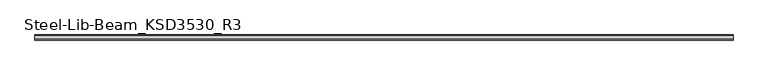
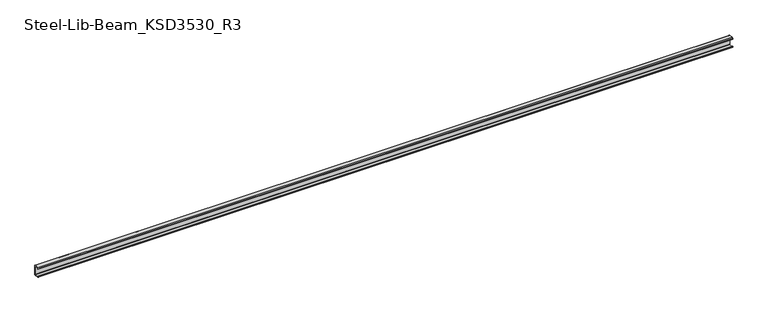
"""IFC4 building model written with IfcOpenShell, lengths in millimetres: beam geometry, Steel-Lib-Beam_KSD3530_R3 : BMS291_C-150×75x20x4.5."""

from ifc_helpers import new_model, si_unit, point, frame, frame_2d, origin, place, context, project, spatial, polyline, circle_curve, trimmed, segment, composite_curve, outline, extrude, source, transform, mapped, element, save


def steel_lib_beam_ksd3530_r3_d49a7bf5(model_context):
    return source(origin(), model_context, "Body", "SweptSolid", [
        extrude(outline(composite_curve([segment(trimmed(circle_curve(frame_2d((-41.0, 66.0)), 9.0), [point((-50.0, 66.0))], [point((-41.0, 75.0))], False, "CARTESIAN"), True, "CONTINUOUS"), segment(polyline([(-41.0, 75.0), (16.0, 75.0)]), True, "CONTINUOUS"), segment(trimmed(circle_curve(frame_2d((16.0, 66.0)), 9.0), [point((16.0, 75.0))], [point((25.0, 66.0))], False, "CARTESIAN"), True, "CONTINUOUS"), segment(polyline([(25.0, 66.0), (25.0, -66.0)]), True, "CONTINUOUS"), segment(trimmed(circle_curve(frame_2d((16.0, -66.0)), 9.0), [point((25.0, -66.0))], [point((16.0, -75.0))], False, "CARTESIAN"), True, "CONTINUOUS"), segment(polyline([(16.0, -75.0), (-41.0, -75.0)]), True, "CONTINUOUS"), segment(trimmed(circle_curve(frame_2d((-41.0, -66.0)), 9.0), [point((-41.0, -75.0))], [point((-50.0, -66.0))], False, "CARTESIAN"), True, "CONTINUOUS"), segment(polyline([(-50.0, -66.0), (-50.0, -55.0), (-45.5, -55.0), (-45.5, -66.0)]), True, "CONTINUOUS"), segment(trimmed(circle_curve(frame_2d((-41.0, -66.0)), 4.5), [point((-45.5, -66.0))], [point((-41.0, -70.5))], True, "CARTESIAN"), True, "CONTINUOUS"), segment(polyline([(-41.0, -70.5), (16.0, -70.5)]), True, "CONTINUOUS"), segment(trimmed(circle_curve(frame_2d((16.0, -66.0)), 4.5), [point((16.0, -70.5))], [point((20.5, -66.0))], True, "CARTESIAN"), True, "CONTINUOUS"), segment(polyline([(20.5, -66.0), (20.5, 66.0)]), True, "CONTINUOUS"), segment(trimmed(circle_curve(frame_2d((16.0, 66.0)), 4.5), [point((20.5, 66.0))], [point((16.0, 70.5))], True, "CARTESIAN"), True, "CONTINUOUS"), segment(polyline([(16.0, 70.5), (-41.0, 70.5)]), True, "CONTINUOUS"), segment(trimmed(circle_curve(frame_2d((-41.0, 66.0)), 4.5), [point((-41.0, 70.5))], [point((-45.5, 66.0))], True, "CARTESIAN"), True, "CONTINUOUS"), segment(polyline([(-45.5, 66.0), (-45.5, 55.0), (-50.0, 55.0), (-50.0, 66.0)]), True, "CONTINUOUS")], self_intersect=False)), frame((-5049.5, 0.0, 0.0), z_axis=(1.0, 0.0, 0.0), x_axis=(0.0, 1.0, 0.0)), (0.0, 0.0, 1.0), 10224.0),
    ])


if __name__ == "__main__":
    model = new_model("IFC4")
    model_context = context("Model", 3, world=origin())
    ifc_project = project(units=[si_unit("LENGTHUNIT", "METRE", prefix="MILLI")], contexts=[model_context])
    site = spatial("IfcSite", under=ifc_project)
    building = spatial("IfcBuilding", under=site)
    placement = place(None, origin())
    steel_lib_beam_ksd3530_r3_shape = steel_lib_beam_ksd3530_r3_d49a7bf5(model_context)
    element("IfcBeam", 1, ObjectType="Steel-Lib-Beam_KSD3530_R3 : BMS291_C-150×75x20x4.5", at=placement, inside=building, context=model_context, shape_type="MappedRepresentation", body=[
        mapped(steel_lib_beam_ksd3530_r3_shape, transform((0.0, 0.0, 0.0), x_axis=(1.0, 0.0, 0.0), y_axis=(0.0, 1.0, 0.0), z_axis=(0.0, 0.0, 1.0))),
    ])
    save(model, "model.ifc")

# Revit data of these elements
# Type "Steel-Lib-Beam_KSD3530_R3 : BMS291_C-150×75x20x4.5"
#   Keynote = "C-150×75x20x4.5"
#   SteelWeight = "Light"
#   x = 0.0250 m
#   t1 = 0.0090 m
#   t = 0.0045 m
#   Surface Area = 0.629834 m²/m
#   Section Area = 13.9688 cm²
#   Mass per Unit Length = 10.9655 kg/m
#   C = 0.0200 m
#   A = 0.0750 m
#   Length [instance default] = 1.5000 m
#   H = 0.1500 m
#   hec_material4 [instance default] = none
#   hec_material3 [instance default] = none
#   hec_material2 [instance default] = none
#   hec_material1 [instance default] = none
#   Structural Material [instance default] = Metal - Steel - Light Gauge
#   Assembly Code = ""
# Element 1 (IfcBeam, "Steel-Lib-Beam_KSD3530_R3 : BMS291_C-150×75x20x4.5")
#   Structural Material = none
# Materials
#   "Metal - Steel - Light Gauge": class "Metal", colour RGB 247 247 247, transparency 0
